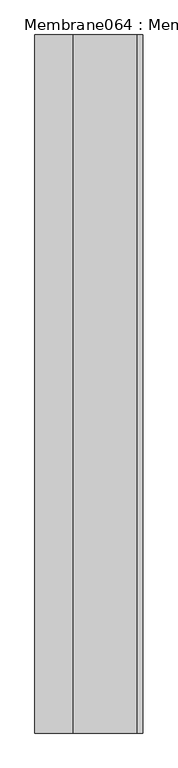
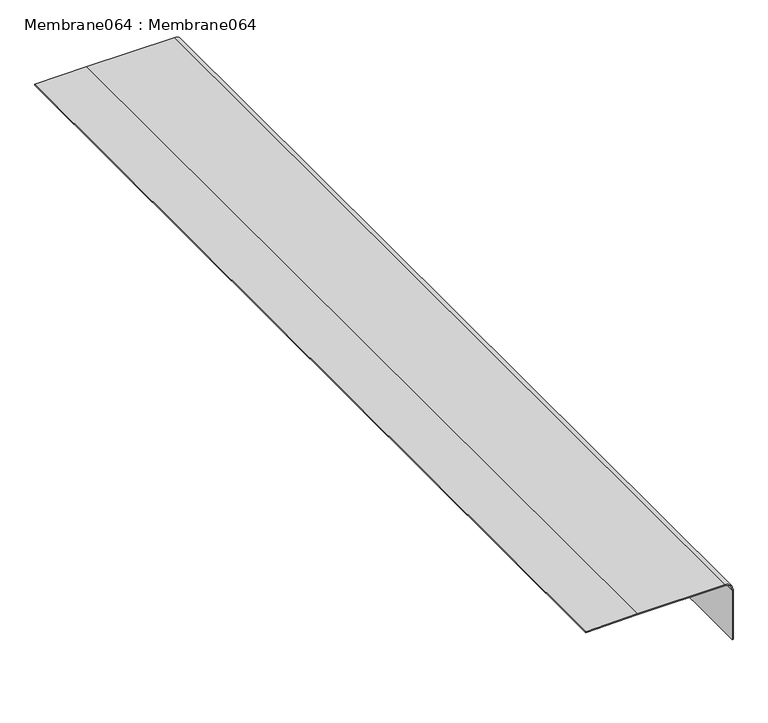
"""IFC4 building model written with IfcOpenShell, lengths in millimetres: proxy geometry, Membrane064 : Membrane064."""

import ifcopenshell
import ifcopenshell.guid

model = None  # the IFC model being written
_history = None  # IfcOwnerHistory: only IFC2X3 demands one
_inside = {}  # id of a spatial element -> (the spatial element, [elements in it])
_under = {}  # id of a project, library or spatial element -> (it, [spatial elements below it])
_declared = {}  # id of a project -> (the project, [libraries it declares])
_typed = {}  # id of a type object -> (the type object, [elements of that type])
_made_of = {}  # id of a material, layer set ... -> (it, [elements and type objects made of it])


def new_model(schema):
    """Start an empty IFC model of exactly this schema.

    Asked for "IFC4X3", IfcOpenShell would pick the latest addendum, in which some entities
    have other attributes; the version numbers below select the first issue.
    IFC2X3 requires an IfcOwnerHistory on every rooted entity: one is made here for all.
    """
    global model, _history
    if schema == "IFC4X3":
        model = ifcopenshell.file(schema_version=(4, 3, 0, 0))
    else:
        model = ifcopenshell.file(schema=schema)
    _inside.clear()
    _under.clear()
    _declared.clear()
    _typed.clear()
    _made_of.clear()
    _history = None
    if model.schema == "IFC2X3":
        org = make("IfcOrganization", Name="unknown")
        user = make(
            "IfcPersonAndOrganization",
            ThePerson=make("IfcPerson", FamilyName="unknown"),
            TheOrganization=org,
        )
        app = make(
            "IfcApplication",
            ApplicationDeveloper=org,
            Version="unknown",
            ApplicationFullName="unknown",
            ApplicationIdentifier="unknown",
        )
        _history = make(
            "IfcOwnerHistory",
            OwningUser=user,
            OwningApplication=app,
            ChangeAction="ADDED",
            CreationDate=0,
        )
    return model


def make(cls, **values):
    """One entity of the class cls with the attributes given. An attribute that is None is left unset."""
    return model.create_entity(
        cls, **{name: value for name, value in values.items() if value is not None}
    )


def rooted(cls, **values):
    """An entity with a GlobalId (a new one), such as an element, a storey or a relation."""
    return make(cls, GlobalId=ifcopenshell.guid.new(), OwnerHistory=_history, **values)


def si_unit(unit_type, name, prefix=None):
    """IfcSIUnit, for example si_unit("LENGTHUNIT", "METRE", prefix="MILLI")."""
    return make("IfcSIUnit", UnitType=unit_type, Prefix=prefix, Name=name)


def assignment(units):
    """IfcUnitAssignment: the units of a project."""
    return None if units is None else make("IfcUnitAssignment", Units=units)


def point(xyz):
    """IfcCartesianPoint."""
    return None if xyz is None else make("IfcCartesianPoint", Coordinates=xyz)


def direction(xyz):
    """IfcDirection."""
    return None if xyz is None else make("IfcDirection", DirectionRatios=xyz)


def frame(location, z_axis=None, x_axis=None):
    """IfcAxis2Placement3D, a coordinate frame: its origin and axes. An axis left out is left unset."""
    return make(
        "IfcAxis2Placement3D",
        Location=point(location),
        Axis=direction(z_axis),
        RefDirection=direction(x_axis),
    )


def frame_2d(location, x_axis=None):
    """IfcAxis2Placement2D, a coordinate frame in the plane: its origin and x axis."""
    return make(
        "IfcAxis2Placement2D", Location=point(location), RefDirection=direction(x_axis)
    )


def origin():
    """The frame at (0, 0, 0) with its axes left unset."""
    return frame((0.0, 0.0, 0.0))


def place(relative_to, where):
    """IfcLocalPlacement: puts the frame where relative to a parent placement (None: the world)."""
    return make(
        "IfcLocalPlacement", PlacementRelTo=relative_to, RelativePlacement=where
    )


def context(
    kind, dimensions, precision=None, world=None, true_north=None, identifier=None
):
    """IfcGeometricRepresentationContext, for example the 3D "Model" context."""
    return make(
        "IfcGeometricRepresentationContext",
        ContextIdentifier=identifier,
        ContextType=kind,
        CoordinateSpaceDimension=dimensions,
        Precision=precision,
        WorldCoordinateSystem=world,
        TrueNorth=true_north,
    )


def project(units=None, contexts=None):
    """IfcProject with its units and contexts."""
    return rooted(
        "IfcProject",
        Name="project",
        RepresentationContexts=contexts,
        UnitsInContext=assignment(units),
    )


def spatial(cls, under=None, at=None, **own):
    """A site, building, storey or space (cls), placed at a placement, below another one or the project."""
    s = rooted(cls, ObjectPlacement=at, **own)
    if under is not None:
        _under.setdefault(under.id(), (under, []))[1].append(s)
    return s


def polyline(points):
    """IfcPolyline through the points."""
    return make("IfcPolyline", Points=[point(p) for p in points])


def circle_curve(where, radius):
    """IfcCircle in the frame where."""
    return make("IfcCircle", Position=where, Radius=radius)


def trimmed(basis, trim1, trim2, sense, master):
    """IfcTrimmedCurve: the piece of a basis curve between two trims."""
    return make(
        "IfcTrimmedCurve",
        BasisCurve=basis,
        Trim1=trim1,
        Trim2=trim2,
        SenseAgreement=sense,
        MasterRepresentation=master,
    )


def segment(curve, same_sense, transition):
    """IfcCompositeCurveSegment."""
    return make(
        "IfcCompositeCurveSegment",
        Transition=transition,
        SameSense=same_sense,
        ParentCurve=curve,
    )


def composite_curve(segments, self_intersect=None):
    """IfcCompositeCurve: segments joined end to end."""
    return make("IfcCompositeCurve", Segments=segments, SelfIntersect=self_intersect)


def outline(outer, holes=None, kind="AREA"):
    """IfcArbitraryClosedProfileDef: a profile drawn as a closed curve; with holes, ...WithVoids."""
    if holes is None:
        return make("IfcArbitraryClosedProfileDef", ProfileType=kind, OuterCurve=outer)
    return make(
        "IfcArbitraryProfileDefWithVoids",
        ProfileType=kind,
        OuterCurve=outer,
        InnerCurves=holes,
    )


def extrude(swept, where, along, depth):
    """IfcExtrudedAreaSolid: the profile swept, set in the frame where, extruded along a direction by depth."""
    return make(
        "IfcExtrudedAreaSolid",
        SweptArea=swept,
        Position=where,
        ExtrudedDirection=direction(along),
        Depth=depth,
    )


def shape(context_of_items, identifier, shape_type, items):
    """IfcShapeRepresentation: the items that make up one representation, for example the "Body"."""
    return make(
        "IfcShapeRepresentation",
        ContextOfItems=context_of_items,
        RepresentationIdentifier=identifier,
        RepresentationType=shape_type,
        Items=items,
    )


def source(mapping_origin, context_of_items, identifier, shape_type, items):
    """IfcRepresentationMap: a shape defined once, which mapped items show again and again."""
    return make(
        "IfcRepresentationMap",
        MappingOrigin=mapping_origin,
        MappedRepresentation=shape(context_of_items, identifier, shape_type, items),
    )


def transform(
    local_origin,
    x_axis=None,
    y_axis=None,
    z_axis=None,
    scale=None,
    scale2=None,
    scale3=None,
    uniform=True,
):
    """IfcCartesianTransformationOperator3D, or its non-uniform kind. x_axis, y_axis, z_axis: its Axis1, 2, 3."""
    if uniform:
        return make(
            "IfcCartesianTransformationOperator3D",
            Axis1=direction(x_axis),
            Axis2=direction(y_axis),
            LocalOrigin=point(local_origin),
            Scale=scale,
            Axis3=direction(z_axis),
        )
    return make(
        "IfcCartesianTransformationOperator3DnonUniform",
        Axis1=direction(x_axis),
        Axis2=direction(y_axis),
        LocalOrigin=point(local_origin),
        Scale=scale,
        Axis3=direction(z_axis),
        Scale2=scale2,
        Scale3=scale3,
    )


def mapped(mapping_source, mapping_target):
    """IfcMappedItem: shows the shape of a source again, moved by a transform."""
    return make(
        "IfcMappedItem", MappingSource=mapping_source, MappingTarget=mapping_target
    )


def made_of(thing, what):
    """Note that an element or type object is made of a material, layer set ...; save() writes the relation."""
    if what is not None:
        _made_of.setdefault(what.id(), (what, []))[1].append(thing)
    return thing


def element(
    cls,
    number,
    at=None,
    inside=None,
    cuts=None,
    type_object=None,
    material=None,
    context=None,
    identifier="Body",
    shape_type=None,
    held_by="IfcProductDefinitionShape",
    body=None,
    shapes=None,
    **own,
):
    """One element of the class cls, such as IfcWall. Its Tag is "e" and its number.

    at: its placement. inside: the storey or other place that contains it. cuts: it is an
    opening in that element (IfcRelVoidsElement). A single representation is given by context,
    identifier, shape_type and body (its items); several are given by shapes. held_by: the class
    of the entity that holds the representations. save() writes the other relations.
    """
    e = rooted(cls, Tag="e%d" % number, ObjectPlacement=at, **own)
    if body is not None:
        shapes = [shape(context, identifier, shape_type, body)]
    if shapes is not None:
        e.Representation = make(held_by, Representations=shapes)
    if inside is not None:
        _inside.setdefault(inside.id(), (inside, []))[1].append(e)
    if cuts is not None:
        rooted(
            "IfcRelVoidsElement", RelatingBuildingElement=cuts, RelatedOpeningElement=e
        )
    if type_object is not None:
        _typed.setdefault(type_object.id(), (type_object, []))[1].append(e)
    return made_of(e, material)


def aggregate(whole, parts):
    """IfcRelAggregates: a whole, such as a stair, and the parts it consists of."""
    return rooted("IfcRelAggregates", RelatingObject=whole, RelatedObjects=parts)


def save(model, path):
    """Write the relations noted so far, then the file.

    IfcRelAggregates (storeys below a building ...), IfcRelContainedInSpatialStructure (elements
    in a storey), IfcRelDefinesByType, IfcRelAssociatesMaterial and IfcRelDeclares: one each for
    every whole, place, type object, material and project.
    """
    for whole, parts in _under.values():
        aggregate(whole, parts)
    for where, things in _inside.values():
        rooted(
            "IfcRelContainedInSpatialStructure",
            RelatedElements=things,
            RelatingStructure=where,
        )
    for kind, things in _typed.values():
        rooted("IfcRelDefinesByType", RelatedObjects=things, RelatingType=kind)
    for what, things in _made_of.values():
        rooted("IfcRelAssociatesMaterial", RelatedObjects=things, RelatingMaterial=what)
    for by, libraries in _declared.values():
        rooted("IfcRelDeclares", RelatingContext=by, RelatedDefinitions=libraries)
    model.write(path)


def membrane064_membrane064_535062ed(model_context):
    return source(origin(), model_context, "Body", "SweptSolid", [
        extrude(outline(composite_curve([segment(polyline([(40234.8417335, -4392.7651271), (40125.2457074, -4392.7651271), (40125.2457074, -4390.7651271), (40234.8417335, -4390.7651271)]), True, "CONTINUOUS"), segment(trimmed(circle_curve(frame_2d((40234.8417335, -4407.7651271)), 17.0), [point((40234.8417335, -4390.7651271))], [point((40251.8417335, -4407.7651271))], False, "CARTESIAN"), True, "CONTINUOUS"), segment(polyline([(40251.8417335, -4407.7651271), (40251.8417335, -4591.7190058), (40250.2861996, -4699.8063764), (40248.2859925, -4699.8063764), (40249.8417335, -4591.7046151), (40249.8417335, -4407.7651271)]), True, "CONTINUOUS"), segment(trimmed(circle_curve(frame_2d((40234.8417335, -4407.7651271)), 15.0), [point((40249.8417335, -4407.7651271))], [point((40234.8417335, -4392.7651271))], True, "CARTESIAN"), True, "CONTINUOUS")], self_intersect=False)), frame((0.0, -1052.8906574, 0.0), z_axis=(0.0, 1.0, 0.0), x_axis=(0.0, 0.0, 1.0)), (0.0, 0.0, 1.0), 2000.0),
    ])


if __name__ == "__main__":
    model = new_model("IFC4")
    model_context = context("Model", 3, world=origin())
    ifc_project = project(units=[si_unit("LENGTHUNIT", "METRE", prefix="MILLI")], contexts=[model_context])
    site = spatial("IfcSite", under=ifc_project)
    building = spatial("IfcBuilding", under=site)
    placement = place(None, origin())
    membrane064_membrane064_shape = membrane064_membrane064_535062ed(model_context)
    element("IfcBuildingElementProxy", 1, Name="Membrane064 : Membrane064", ObjectType="Membrane064 : Membrane064", at=placement, inside=building, context=model_context, shape_type="MappedRepresentation", body=[
        mapped(membrane064_membrane064_shape, transform((0.0, 0.0, 0.0), x_axis=(1.0, 0.0, 0.0), y_axis=(0.0, 1.0, 0.0), z_axis=(0.0, 0.0, 1.0))),
    ])
    save(model, "model.ifc")

# Revit data of these elements
# Type "Membrane064 : Membrane064"
#   NameOverride = "Membrane064"
# Element 1 (IfcBuildingElementProxy, "Membrane064 : Membrane064")
#   Materials on its faces: "THREE PLY BUILT UP ROOF MEMBRANE"
# Materials
#   "THREE PLY BUILT UP ROOF MEMBRANE": class "Unassigned", colour RGB 63 63 63, transparency 0
